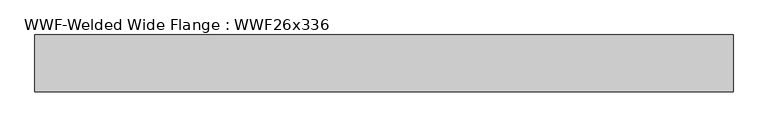
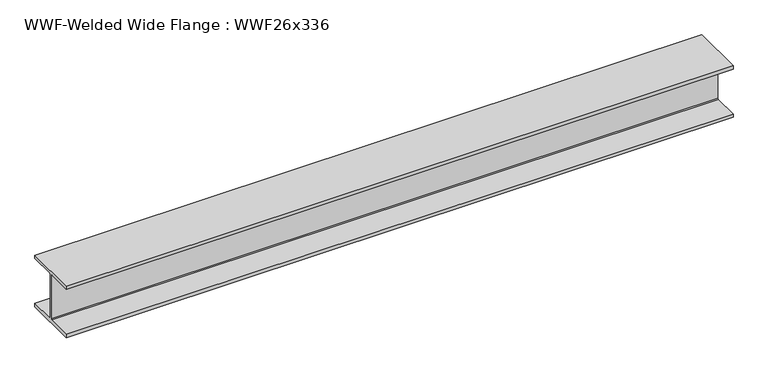
"""IFC4 building model written with IfcOpenShell, lengths in millimetres: beam geometry, WWF-Welded Wide Flange : WWF26x336."""

from ifc_helpers import new_model, si_unit, frame, origin, place, context, project, spatial, polyline, outline, extrude, source, transform, mapped, element, save


def wwf_welded_wide_flange_wwf26x336_e1246b3c(model_context):
    return source(origin(), model_context, "Body", "SweptSolid", [
        extrude(outline(polyline([(324.993, -284.988), (324.993, -324.993), (-324.993, -324.993), (-324.993, -284.988), (-20.6375, -284.988), (-9.9949, -274.3454), (-9.9949, 274.3454), (-20.6375, 284.988), (-324.993, 284.988), (-324.993, 324.993), (324.993, 324.993), (324.993, 284.988), (20.6375, 284.988), (9.9949, 274.3454), (9.9949, -274.3454), (20.6375, -284.988), (324.993, -284.988)])), frame((-3934.8877112, 0.0, 0.0), z_axis=(1.0, 0.0, 0.0), x_axis=(0.0, 1.0, 0.0)), (0.0, 0.0, 1.0), 7999.1216255),
    ])


if __name__ == "__main__":
    model = new_model("IFC4")
    model_context = context("Model", 3, world=origin())
    ifc_project = project(units=[si_unit("LENGTHUNIT", "METRE", prefix="MILLI")], contexts=[model_context])
    site = spatial("IfcSite", under=ifc_project)
    building = spatial("IfcBuilding", under=site)
    placement = place(None, origin())
    wwf_welded_wide_flange_wwf26x336_shape = wwf_welded_wide_flange_wwf26x336_e1246b3c(model_context)
    element("IfcBeam", 1, ObjectType="WWF-Welded Wide Flange : WWF26x336", at=placement, inside=building, context=model_context, shape_type="MappedRepresentation", body=[
        mapped(wwf_welded_wide_flange_wwf26x336_shape, transform((0.0, 0.0, 0.0), x_axis=(1.0, 0.0, 0.0), y_axis=(0.0, 1.0, 0.0), z_axis=(0.0, 0.0, 1.0))),
    ])
    save(model, "model.ifc")

# Revit data of these elements
# Type "WWF-Welded Wide Flange : WWF26x336"
#   Assembly Code = "B10"
#   Nominal d = "12"
#   W = 336
#   Length [instance default] = 1524 mm
#   bf = 649.986 mm
#   d = 649.986 mm
#   k = 20.638 mm
#   tf = 40.005 mm
#   tw = 19.99 mm
#   A = 0.0635483 m²
#   Structural Material [instance default] = Steel ASTM A572
# Element 1 (IfcBeam, "WWF-Welded Wide Flange : WWF26x336")
#   Structural Material = Metal - Steel 43-275
#   Materials on its faces: "Metal - Steel 43-275"
# Materials
#   "Steel ASTM A572": class "Metal", colour RGB 247 247 247, transparency 0, Description = "Structural steel, high strength low alloy, ASTM - A572 - 50", Cost = 0
#   "Metal - Steel 43-275": class "Metal", colour RGB 247 247 247, transparency 0, Cost = 0
